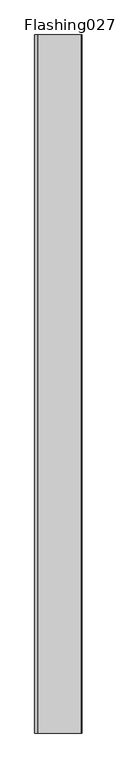
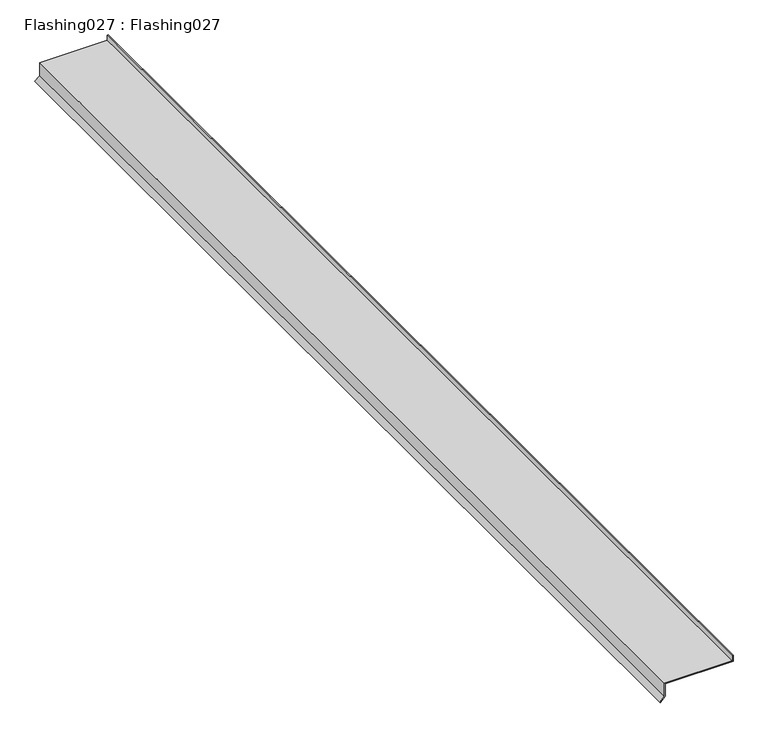
"""IFC4 building model written with IfcOpenShell, lengths in millimetres: proxy geometry, Flashing027 : Flashing027."""

from ifc_helpers import new_model, si_unit, frame, origin, place, context, project, spatial, polyline, outline, extrude, source, transform, mapped, element, save


def flashing027_flashing027_c57af108(model_context):
    return source(origin(), model_context, "Body", "SweptSolid", [
        extrude(outline(polyline([(40335.3398438, -986.5449829), (40325.640625, -986.5449829), (40325.640625, -1111.5771484), (40300.3872772, -1111.5771484), (40291.9157249, -1120.4555041), (40290.46875, -1119.0748291), (40299.53125, -1109.5771484), (40323.640625, -1109.5771484), (40323.640625, -984.5449829), (40335.3398438, -984.5449829), (40335.3398438, -986.5449829)])), frame((0.0, -1052.8906574, 0.0), z_axis=(0.0, 1.0, 0.0), x_axis=(0.0, 0.0, 1.0)), (0.0, 0.0, 1.0), 2000.0),
    ])


if __name__ == "__main__":
    model = new_model("IFC4")
    model_context = context("Model", 3, world=origin())
    ifc_project = project(units=[si_unit("LENGTHUNIT", "METRE", prefix="MILLI")], contexts=[model_context])
    site = spatial("IfcSite", under=ifc_project)
    building = spatial("IfcBuilding", under=site)
    placement = place(None, origin())
    flashing027_flashing027_shape = flashing027_flashing027_c57af108(model_context)
    element("IfcBuildingElementProxy", 1, Name="Flashing027 : Flashing027", ObjectType="Flashing027 : Flashing027", at=placement, inside=building, context=model_context, shape_type="MappedRepresentation", body=[
        mapped(flashing027_flashing027_shape, transform((0.0, 0.0, 0.0), x_axis=(1.0, 0.0, 0.0), y_axis=(0.0, 1.0, 0.0), z_axis=(0.0, 0.0, 1.0))),
    ])
    save(model, "model.ifc")

# Revit data of these elements
# Type "Flashing027 : Flashing027"
#   NameOverride = "Flashing027"
# Element 1 (IfcBuildingElementProxy, "Flashing027 : Flashing027")
#   Materials on its faces: "COPPER SILL PAN AT ALL EXTERIOR WINDOWS/DOORS PER DETAIL 1/A4.1"
# Materials
#   "COPPER SILL PAN AT ALL EXTERIOR WINDOWS/DOORS PER DETAIL 1/A4.1": class "Unassigned", colour RGB 255 170 255, transparency 0, Cost = 0
